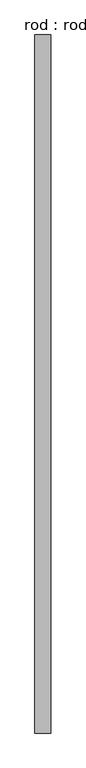
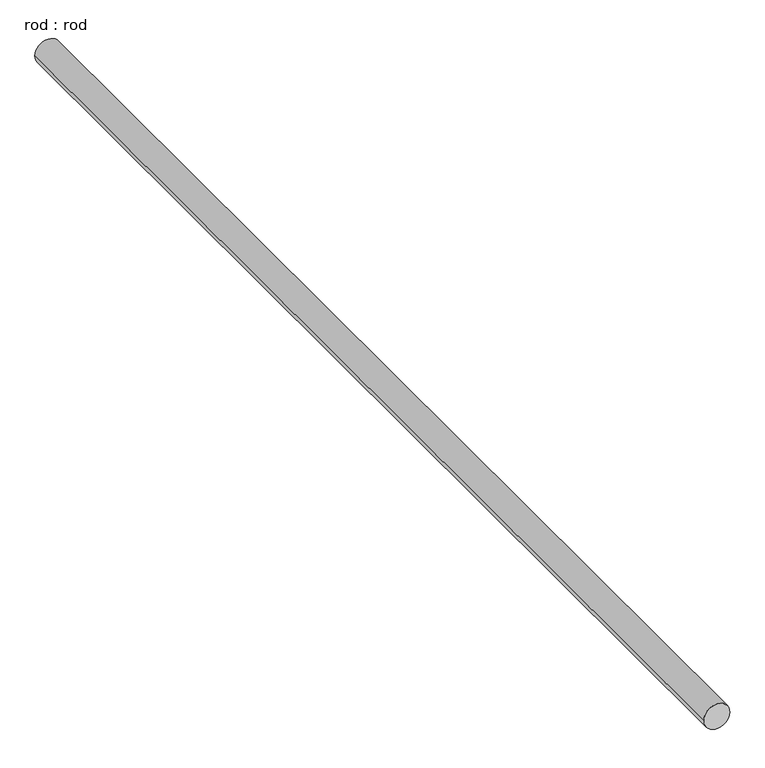
"""IFC4 building model written with IfcOpenShell, lengths in millimetres: proxy geometry, rod : rod."""

from ifc_helpers import new_model, si_unit, point, frame, frame_2d, origin, place, context, project, spatial, circle_curve, trimmed, segment, composite_curve, outline, extrude, source, transform, mapped, element, save


def rod_rod_ade6102d(model_context):
    return source(origin(), model_context, "Body", "SweptSolid", [
        extrude(outline(composite_curve([segment(trimmed(circle_curve(frame_2d((0.0108462, 0.0)), 200.0), [point((0.0108462, 200.0))], [point((0.0108462, -200.0))], False, "CARTESIAN"), True, "CONTINUOUS"), segment(trimmed(circle_curve(frame_2d((0.0108462, 0.0)), 200.0), [point((0.0108462, -200.0))], [point((0.0108462, 200.0))], False, "CARTESIAN"), True, "CONTINUOUS")], self_intersect=False)), frame((0.0, -4757.2713847, 0.0), z_axis=(0.0, 1.0, 0.0), x_axis=(0.0, 0.0, 1.0)), (0.0, 0.0, 1.0), 17700.0),
    ])


if __name__ == "__main__":
    model = new_model("IFC4")
    model_context = context("Model", 3, world=origin())
    ifc_project = project(units=[si_unit("LENGTHUNIT", "METRE", prefix="MILLI")], contexts=[model_context])
    site = spatial("IfcSite", under=ifc_project)
    building = spatial("IfcBuilding", under=site)
    placement = place(None, origin())
    rod_rod_shape = rod_rod_ade6102d(model_context)
    element("IfcBuildingElementProxy", 1, Name="rod : rod", ObjectType="rod : rod", at=placement, inside=building, context=model_context, shape_type="MappedRepresentation", body=[
        mapped(rod_rod_shape, transform((0.0, 0.0, 0.0), x_axis=(1.0, 0.0, 0.0), y_axis=(0.0, 1.0, 0.0), z_axis=(0.0, 0.0, 1.0))),
    ])
    save(model, "model.ifc")

# Revit data of these elements
# Type "rod : rod"
#   Default Elevation = 0
